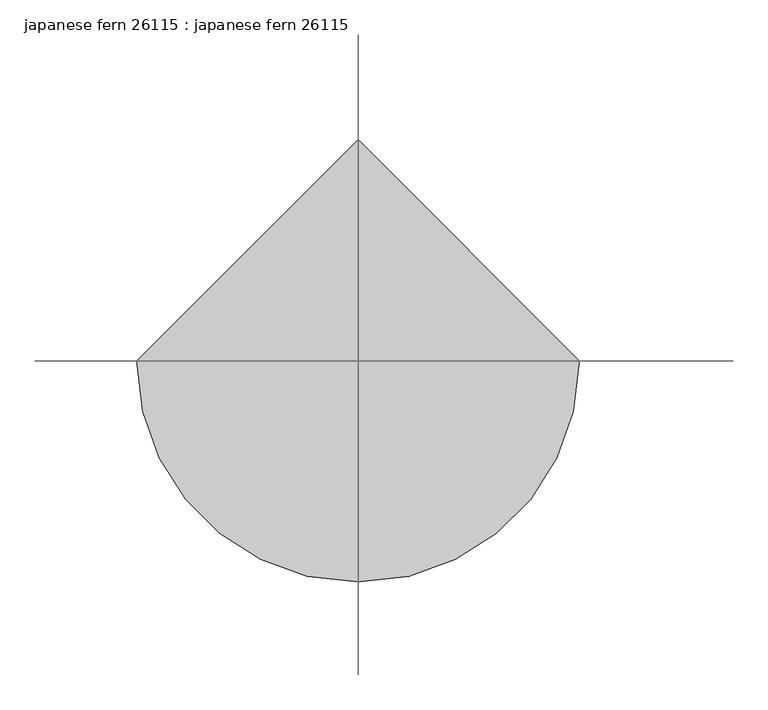
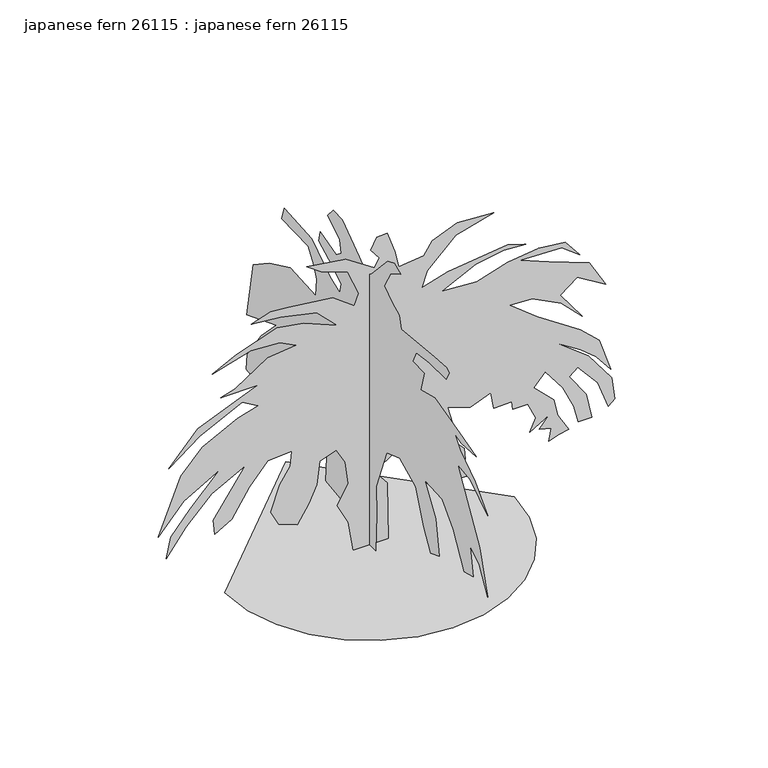
"""IFC4 building model written with IfcOpenShell, lengths in millimetres: proxy geometry, japanese fern 26115 : japanese fern 26115."""

from ifc_helpers import new_model, si_unit, origin, place, context, project, spatial, triangles, source, transform, mapped, element, save


def japanese_fern_26115_japanese_fern_26115_30b4c15b(model_context):
    return source(origin(), model_context, "Body", "Tessellation", [
        triangles([(-340.212337, 0.0, 2.34e-05), (-331.2181912, -77.9542988, 2.34e-05), (-305.6048564, -149.5428615, 2.34e-05), (-265.4195731, -212.7146324, 2.34e-05), (-212.7146324, -265.4195731, 2.34e-05), (-149.5428615, -305.6048564, 2.34e-05), (-77.9542988, -331.2181912, 2.34e-05), (1.49e-05, -340.212337, 2.34e-05), (77.9542988, -331.2181912, 2.34e-05), (149.5428615, -305.6048564, 2.34e-05), (212.7146324, -265.4195731, 2.34e-05), (265.4195731, -212.7146324, 2.34e-05), (305.6048564, -149.5428615, 2.34e-05), (331.2181912, -77.9542988, 2.34e-05), (340.212337, 2.97e-05, 2.34e-05), (-4.46e-05, 340.212337, 2.34e-05), (-37.8980319, 2.29e-05, 3.6e-06), (-50.0874814, 2.41e-05, 73.5418183), (-75.8826774, 2.22e-05, 123.7339445), (-49.5540792, 1.83e-05, 170.5209506), (-56.979003, 1.53e-05, 225.9335385), (-77.3492758, 1.4e-05, 262.2445852), (-116.2627981, 1.66e-05, 248.3474865), (-123.5028085, 2.02e-05, 192.7652324), (-143.0648503, 2.35e-05, 151.8270789), (-169.0734009, 2.72e-05, 109.3715308), (-213.7047246, 2.81e-05, 126.2541304), (-232.5443813, 2.67e-05, 163.0480237), (-210.7659323, 2.22e-05, 223.3318078), (-185.9735321, 1.89e-05, 260.6164324), (-182.3167059, 1.66e-05, 296.5396212), (-238.5613832, 1.93e-05, 292.8185184), (-282.7321973, 2.42e-05, 242.1521888), (-323.5728004, 2.99e-05, 177.126216), (-363.5396922, 3.3e-05, 153.4968807), (-367.1566226, 3.1e-05, 190.2732333), (-291.3732759, 2.12e-05, 298.3785896), (-370.9310652, 2.72e-05, 256.7835813), (-430.3492407, 3.34e-05, 195.5366293), (-477.8725754, 3.92e-05, 133.2528402), (-467.4636904, 3.58e-05, 182.8625483), (-420.8344145, 3.05e-05, 237.2243282), (-351.5280344, 2.32e-05, 310.1438599), (-436.732245, 2.98e-05, 261.3606638), (-497.0571965, 3.65e-05, 192.7571115), (-443.5089389, 2.62e-05, 326.4709519), (-392.9096655, 2.08e-05, 380.0648827), (-309.8949288, 1.46e-05, 423.094996), (-260.7967811, 1.16e-05, 437.3545544), (-299.3412489, 1.2e-05, 459.500768), (-398.9192914, 1.93e-05, 409.5872812), (-471.8705798, 2.58e-05, 354.6903414), (-403.1941031, 1.83e-05, 430.1180775), (-300.6061608, 1.12e-05, 473.1100754), (-262.5823916, 8.7e-06, 488.4237482), (-349.0058046, 1.24e-05, 488.2357873), (-315.6607106, 1.04e-05, 498.3805169), (-238.5613832, 4e-06, 548.5353044), (-172.4069002, 6e-07, 556.9452561), (-210.7659323, 1.1e-06, 576.3305191), (-278.7875798, 3.9e-06, 580.4732532), (-369.1987945, 9.4e-06, 554.0953574), (-313.0699167, 5.2e-06, 582.9446503), (-216.6861742, -1e-06, 616.0738781), (-154.0988607, -3.1e-06, 605.5227053), (-75.0741966, -4.5e-06, 572.1420393), (-123.4916265, -5.3e-06, 620.6382071), (-209.0953766, -2.7e-06, 638.8728498), (-277.4743968, -1e-07, 645.8171934), (-232.2393309, -3e-06, 661.5423237), (-190.0088236, -4.6e-06, 657.7145777), (-85.7208487, -8.4e-06, 644.6056395), (-35.6564855, -8.3e-06, 606.9044523), (-24.5384073, -1.05e-05, 634.6996307), (-50.8667489, -1.3e-05, 696.1980572), (-113.4009815, -1.16e-05, 718.2401711), (-146.8372491, -1.16e-05, 743.1016623), (-55.5814956, -1.48e-05, 730.2366045), (11.5952668, -1.5e-05, 684.7325506), (23.1518731, -1.68e-05, 706.0913486), (3.2567592, -1.75e-05, 731.9840996), (17.6289544, -1.97e-05, 758.3441912), (41.4979712, -2.09e-05, 760.5615704), (59.6452374, -1.86e-05, 708.9971306), (68.5156716, -1.65e-05, 668.0955574), (127.4710438, -1.95e-05, 674.2321741), (147.7915331, -2.21e-05, 704.1889212), (206.1616894, -2.62e-05, 729.2028013), (292.3257614, -2.96e-05, 723.6452917), (202.8348031, -2.42e-05, 698.6847513), (136.1791696, -1.75e-05, 634.3440565), (123.7575623, -1.46e-05, 595.466851), (183.9252741, -1.84e-05, 615.2432602), (325.6810292, -2.56e-05, 631.9208759), (367.486835, -2.67e-05, 619.3809437), (315.6911957, -2.46e-05, 622.1876038), (249.7079049, -2.1e-05, 609.8203354), (170.7500609, -1.52e-05, 570.6967787), (252.258585, -1.85e-05, 566.1527246), (325.6530876, -2.3e-05, 588.2608592), (397.9490381, -2.68e-05, 598.5656445), (460.1815041, -2.91e-05, 591.0853598), (495.2309272, -2.81e-05, 548.5353044), (452.9501141, -2.81e-05, 580.5189626), (355.0433722, -2.4e-05, 583.2977174), (420.1841635, -2.53e-05, 556.8741122), (516.8336057, -2.73e-05, 520.4505724), (556.2848313, -2.51e-05, 453.460657), (489.3051261, -2.46e-05, 494.41557), (449.4220591, -2.1e-05, 463.6816175), (500.7909802, -1.9e-05, 392.8817239), (450.7580967, -1.98e-05, 442.9146074), (383.0951119, -1.89e-05, 477.7430411), (329.99392, -1.68e-05, 480.9358332), (395.1677399, -1.66e-05, 429.0157465), (495.6652757, -1.69e-05, 361.8734422), (541.06265, -1.64e-05, 319.2167072), (567.5802175, -1.27e-05, 237.3833302), (533.9328526, -1.38e-05, 280.9008592), (497.6007317, -1.4e-05, 310.7127932), (440.194243, -1.36e-05, 346.6664852), (514.6872977, -1.35e-05, 290.0397636), (570.595186, -1.15e-05, 215.9856355), (576.6531012, -8.5e-06, 161.5684811), (561.938883, -7.1e-06, 148.2847988), (536.9249665, -1e-05, 214.9932542), (489.6734176, -1.12e-05, 270.583393), (469.5464848, -9.4e-06, 254.0962635), (510.5775922, -7.7e-06, 195.5264555), (523.0261056, -4.6e-06, 134.3872005), (491.7079591, -3.2e-06, 133.6020922), (481.1339315, -5.3e-06, 176.3159639), (454.7662096, -7.4e-06, 231.6510674), (413.5344604, -8.8e-06, 285.1248746), (386.501263, -5.8e-06, 255.5745526), (434.0830244, -5.2e-06, 209.4342185), (443.1813063, -3e-06, 166.6068182), (468.6523896, -1.6e-06, 123.9640722), (446.3842358, -3e-07, 118.289464), (421.5049404, 1.3e-06, 110.591996), (428.004798, -8e-07, 139.9015351), (399.5416008, 0.0, 147.6790127), (422.9629183, -2.7e-06, 176.0799863), (377.2150203, 9e-07, 148.592647), (391.2256476, -1.5e-06, 179.1531272), (372.9656067, -3.1e-06, 218.8891102), (336.6588839, -1.5e-06, 219.0854463), (334.8783603, -2.6e-06, 238.301043), (292.3257614, -6e-07, 237.2294151), (285.8309907, -2.8e-06, 277.7512695), (236.7361495, 5e-07, 259.4658122), (183.9252741, 1.8e-06, 276.1434461), (200.6023993, 4.7e-06, 214.9932542), (199.418242, 6.4e-06, 187.1818159), (222.8385421, 6.9e-06, 162.1823971), (225.6180599, 8.4e-06, 134.3872005), (208.5548754, 9.9e-06, 121.5754553), (237.8440942, 1.05e-05, 90.4480402), (182.0385615, 1.28e-05, 92.8412262), (191.5158174, 1e-05, 133.3458033), (165.4579784, 1e-05, 152.2179799), (173.5882597, 8.2e-06, 176.3515177), (109.0494575, 1.14e-05, 169.6062899), (94.9809212, 1.06e-05, 192.7571115), (145.0122605, 6.8e-06, 220.5522899), (83.3228392, 9.3e-06, 223.7369429), (11.6764698, 1.52e-05, 177.2189248), (42.170055, 1.61e-05, 139.9462362), (44.9495728, 1.82e-05, 0.0), (0.00212, 26.6938489, 3.6e-06), (0.0021253, 22.2078332, 125.235588), (0.0021271, 60.1697466, 128.8281648), (0.002126, 119.4035039, 42.9622804), (0.0021289, 177.9956579, 51.1230378), (0.0021314, 173.4581986, 113.1355544), (0.0021337, 137.5657583, 202.421547), (0.0021299, 136.57414, 252.5593115), (0.0021317, 167.407932, 262.8744886), (0.0021371, 226.3958104, 190.2732333), (0.0021373, 288.3557457, 133.4656906), (0.0021388, 315.632769, 140.3605096), (0.0021407, 309.8923854, 190.0641981), (0.0021433, 346.6360002, 212.5124464), (0.0021443, 409.4094941, 172.1231784), (0.0021442, 453.2701527, 125.235588), (0.0021466, 501.6723581, 132.7981805), (0.0021481, 497.133391, 172.1231784), (0.0021432, 441.1721629, 252.2857635), (0.0021433, 378.8939512, 316.9053294), (0.0021465, 498.6472157, 270.4360728), (0.0021515, 472.2337844, 410.5144049), (0.0021506, 407.8956694, 453.4479761), (0.0021486, 323.1969149, 492.7747544), (0.0021437, 217.6417118, 487.9487409), (0.0021455, 214.2957677, 530.5851645), (0.0021473, 226.9167634, 559.1017015), (0.0021497, 249.3380874, 591.8626016), (0.0021545, 357.9821463, 594.1105021), (0.0021554, 347.3954378, 625.8731346), (0.0021502, 235.3830889, 618.7560545), (0.0021449, 161.3091401, 570.0389337), (0.0021424, 119.7014417, 554.0699593), (0.0021433, 115.4461873, 579.5537599), (0.0021468, 165.8956152, 609.2361777), (0.0021495, 206.7331843, 630.4121017), (0.0021444, 199.1706008, 657.6358034), (0.0021408, 134.2553771, 640.0184195), (0.0021406, 114.4705746, 656.1245584), (0.0021422, 120.4276329, 685.149095), (0.0021457, 170.4330744, 716.6247173), (0.0021458, 147.7455603, 742.3371014), (0.0021442, 111.4454322, 740.823313), (0.002139, 41.6899925, 691.1155186), (0.0021365, 10.7464246, 665.9695244), (0.0021362, -10.1176737, 680.5009048), (0.0021365, -74.5923583, 749.8987038), (0.0021358, -101.8173226, 761.9992733), (0.0021341, -127.5299701, 749.8987038), (0.0021349, -87.1447716, 726.4240465), (0.002134, -60.7928054, 680.9606152), (0.0021316, -92.5270285, 657.5951809), (0.0021298, -121.8045655, 644.2526087), (0.0021341, -129.7537351, 615.210268), (0.0021228, -265.1681168, 628.8983133), (0.0021208, -315.0816035, 631.9234194), (0.00212, -325.668312, 624.3618896), (0.0021255, -313.5677788, 601.6746117), (0.0021285, -243.6485001, 600.9557965), (0.0021305, -191.8444855, 593.8259992), (0.0021298, -176.5968879, 563.282551), (0.0021277, -223.3409642, 562.4341653), (0.0021262, -209.0156213, 512.3124063), (0.0021243, -266.6794162, 527.5625656), (0.0021188, -366.5470304, 501.9288832), (0.002115, -434.5681692, 482.1855025), (0.0021175, -375.2998755, 480.0595058), (0.002119, -348.4190672, 487.3848581), (0.0021168, -370.0115719, 459.7014462), (0.0021124, -430.801357, 418.7795254), (0.0021078, -482.9678312, 365.7240792), (0.0021129, -410.4102324, 411.3017841), (0.0021154, -360.3773852, 417.8549815), (0.0021108, -398.4519507, 351.1901917), (0.0021049, -449.6938448, 265.8970875), (0.0021049, -481.8349789, 162.1823971), (0.002103, -448.18002, 222.0356478), (0.0021056, -410.473746, 244.4529204), (0.0021022, -423.4226649, 177.6834858), (0.0021093, -387.3318446, 167.7414328), (0.0021087, -342.3053052, 246.2357331), (0.0021128, -296.4634267, 293.7202257), (0.0021161, -226.1207364, 298.3785896), (0.0021111, -271.2183834, 229.5982494), (0.0021128, -284.3374772, 144.5642138), (0.0021137, -249.3695898, 130.0336417), (0.002117, -221.7963819, 179.3619262), (0.002116, -188.1828268, 259.1153067), (0.0021202, -123.9887073, 290.1007337), (0.0021217, -70.0716722, 271.1447323), (0.0021248, -27.498267, 162.3606929), (0.0021217, -30.4360283, 94.6027103), (0.0021177, -25.7012178, 2.43e-05)], [[15, 16, 1], [14, 15, 1], [14, 1, 2], [13, 14, 2], [13, 2, 3], [13, 3, 4], [12, 13, 4], [11, 12, 4], [11, 4, 5], [11, 5, 6], [11, 6, 7], [11, 7, 8], [11, 8, 9], [11, 9, 10], [110, 111, 112], [51, 52, 53], [61, 62, 63], [102, 103, 104], [94, 95, 96], [55, 56, 57], [88, 89, 90], [44, 45, 46], [117, 118, 119], [61, 63, 64], [68, 69, 70], [39, 40, 41], [107, 108, 109], [76, 77, 78], [39, 41, 42], [75, 76, 78], [38, 39, 42], [38, 42, 43], [60, 61, 64], [143, 144, 145], [93, 94, 96], [93, 96, 97], [93, 97, 98], [68, 70, 71], [37, 38, 43], [55, 57, 58], [157, 158, 159], [157, 159, 160], [75, 78, 79], [92, 93, 98], [74, 75, 79], [67, 68, 71], [67, 71, 72], [110, 112, 113], [139, 140, 141], [87, 88, 90], [87, 90, 91], [86, 87, 91], [117, 119, 120], [116, 117, 120], [116, 120, 121], [115, 116, 121], [101, 102, 104], [101, 104, 105], [100, 101, 105], [106, 107, 109], [34, 35, 36], [141, 142, 143], [43, 44, 46], [43, 46, 47], [124, 125, 126], [123, 124, 126], [122, 123, 126], [122, 126, 127], [34, 36, 37], [33, 34, 37], [32, 33, 37], [60, 64, 65], [59, 60, 65], [137, 138, 139], [137, 139, 141], [137, 141, 143], [136, 137, 143], [121, 122, 127], [50, 51, 53], [50, 53, 54], [66, 67, 72], [66, 72, 73], [106, 109, 110], [106, 110, 113], [129, 130, 131], [129, 131, 132], [129, 132, 133], [128, 129, 133], [128, 133, 134], [43, 47, 48], [37, 43, 48], [105, 106, 113], [105, 113, 114], [100, 105, 114], [99, 100, 114], [59, 65, 66], [163, 164, 165], [162, 163, 165], [168, 169, 17], [168, 17, 18], [168, 18, 19], [168, 19, 20], [167, 168, 20], [167, 20, 21], [146, 147, 148], [121, 127, 128], [121, 128, 134], [85, 86, 91], [148, 149, 150], [37, 48, 49], [32, 37, 49], [31, 32, 49], [85, 91, 92], [25, 26, 27], [25, 27, 28], [25, 28, 29], [24, 25, 29], [24, 29, 30], [23, 24, 30], [23, 30, 31], [136, 143, 145], [135, 136, 145], [135, 145, 146], [135, 146, 148], [82, 83, 84], [81, 82, 84], [80, 81, 84], [80, 84, 85], [79, 80, 85], [50, 54, 55], [49, 50, 55], [160, 161, 162], [156, 157, 160], [155, 156, 160], [155, 160, 162], [154, 155, 162], [154, 162, 165], [153, 154, 165], [152, 153, 165], [74, 79, 85], [74, 85, 92], [73, 74, 92], [166, 167, 21], [55, 58, 59], [166, 21, 22], [152, 165, 166], [135, 148, 150], [134, 135, 150], [121, 134, 150], [115, 121, 150], [114, 115, 150], [114, 150, 151], [114, 151, 152], [99, 114, 152], [98, 99, 152], [98, 152, 166], [98, 166, 22], [92, 98, 22], [73, 92, 22], [66, 73, 22], [59, 66, 22], [55, 59, 22], [49, 55, 22], [31, 49, 22], [23, 31, 22], [244, 245, 246], [239, 240, 241], [234, 235, 236], [234, 236, 237], [233, 234, 237], [238, 239, 241], [238, 241, 242], [217, 218, 219], [216, 217, 219], [189, 190, 191], [244, 246, 247], [215, 216, 219], [215, 219, 220], [197, 198, 199], [197, 199, 200], [230, 231, 232], [189, 191, 192], [209, 210, 211], [209, 211, 212], [209, 212, 213], [208, 209, 213], [197, 200, 201], [196, 197, 201], [195, 196, 201], [243, 244, 247], [262, 170, 171], [261, 262, 171], [260, 261, 171], [205, 206, 207], [204, 205, 207], [203, 204, 207], [185, 186, 187], [184, 185, 187], [184, 187, 188], [183, 184, 188], [183, 188, 189], [173, 174, 175], [172, 173, 175], [172, 175, 176], [247, 248, 249], [247, 249, 250], [243, 247, 250], [243, 250, 251], [242, 243, 251], [254, 255, 256], [253, 254, 256], [253, 256, 257], [252, 253, 257], [225, 226, 227], [224, 225, 227], [224, 227, 228], [223, 224, 228], [223, 228, 229], [223, 229, 230], [180, 181, 182], [179, 180, 182], [189, 192, 193], [189, 193, 194], [252, 257, 258], [203, 207, 208], [242, 251, 252], [208, 213, 214], [203, 208, 214], [183, 189, 194], [182, 183, 194], [179, 182, 194], [178, 179, 194], [177, 178, 194], [195, 201, 202], [194, 195, 202], [177, 194, 202], [237, 238, 242], [237, 242, 252], [233, 237, 252], [232, 233, 252], [232, 252, 258], [230, 232, 258], [230, 258, 259], [223, 230, 259], [221, 222, 223], [221, 223, 259], [220, 221, 259], [215, 220, 259], [214, 215, 259], [203, 214, 259], [202, 203, 259], [177, 202, 259], [177, 259, 260], [176, 177, 260], [172, 176, 260], [172, 260, 171]], closed=False),
    ])


if __name__ == "__main__":
    model = new_model("IFC4")
    model_context = context("Model", 3, world=origin())
    ifc_project = project(units=[si_unit("LENGTHUNIT", "METRE", prefix="MILLI")], contexts=[model_context])
    site = spatial("IfcSite", under=ifc_project)
    building = spatial("IfcBuilding", under=site)
    placement = place(None, origin())
    japanese_fern_26115_japanese_fern_26115_shape = japanese_fern_26115_japanese_fern_26115_30b4c15b(model_context)
    element("IfcBuildingElementProxy", 1, Name="japanese fern 26115 : japanese fern 26115", ObjectType="japanese fern 26115 : japanese fern 26115", at=placement, inside=building, context=model_context, shape_type="MappedRepresentation", body=[
        mapped(japanese_fern_26115_japanese_fern_26115_shape, transform((0.0, 0.0, 0.0), x_axis=(1.0, 0.0, 0.0), y_axis=(0.0, 1.0, 0.0), z_axis=(0.0, 0.0, 1.0))),
    ])
    save(model, "model.ifc")

# Revit data of these elements
# Type "japanese fern 26115 : japanese fern 26115"
#   built-in parameter 1005195 = "RPC-16-G1GK-JAPX-7J4P-Q000-ST1L-LVER-AU"
#   Height = 0
